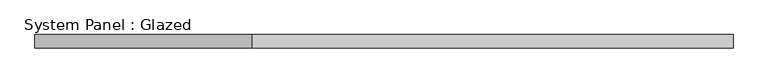
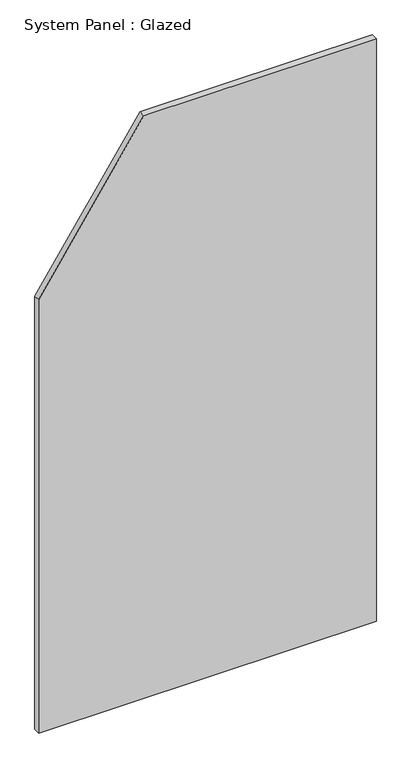
"""IFC4 building model written with IfcOpenShell, lengths in millimetres: plate geometry, System Panel : Glazed."""

from ifc_helpers import new_model, si_unit, frame, origin, place, context, project, spatial, polyline, outline, extrude, source, transform, mapped, element, save


def system_panel_glazed_b9bea58e(model_context):
    return source(origin(), model_context, "Body", "SweptSolid", [
        extrude(outline(polyline([(0.0, -658.3333334), (0.0, 658.3333334), (2400.0, 658.3333334), (2400.0, -248.1683577), (1784.8371088, -658.3333334), (0.0, -658.3333334)])), frame((0.0, 24.5, 0.0), z_axis=(0.0, 1.0, 0.0), x_axis=(0.0, 0.0, 1.0)), (0.0, 0.0, 1.0), 25.0),
    ])


if __name__ == "__main__":
    model = new_model("IFC4")
    model_context = context("Model", 3, world=origin())
    ifc_project = project(units=[si_unit("LENGTHUNIT", "METRE", prefix="MILLI")], contexts=[model_context])
    site = spatial("IfcSite", under=ifc_project)
    building = spatial("IfcBuilding", under=site)
    placement = place(None, origin())
    system_panel_glazed_shape = system_panel_glazed_b9bea58e(model_context)
    element("IfcPlate", 1, ObjectType="System Panel : Glazed", at=placement, inside=building, context=model_context, shape_type="MappedRepresentation", body=[
        mapped(system_panel_glazed_shape, transform((0.0, 0.0, 0.0), x_axis=(1.0, 0.0, 0.0), y_axis=(0.0, 1.0, 0.0), z_axis=(0.0, 0.0, 1.0))),
    ])
    save(model, "model.ifc")

# Revit data of these elements
# Type "System Panel : Glazed"
#   Keynote = "H11"
#   Construction Type Id = "GSP4R"
#   Analytic Construction = "1/8 in Pilkington single glazing"
#   Visual Light Transmittance = 0.9
#   Solar Heat Gain Coefficient = 0.86
#   Heat Transfer Coefficient (U) = 6.7069 W/(m²·K)
#   Define Thermal Properties by = 1
# Element 1 (IfcPlate, "System Panel : Glazed")
#   Materials on its faces: "Glass"
# Materials
#   "Glass": class "Glass", colour RGB 0 128 192, transparency 0.9, Description = "Soda Lime Glass", Cost = 0
